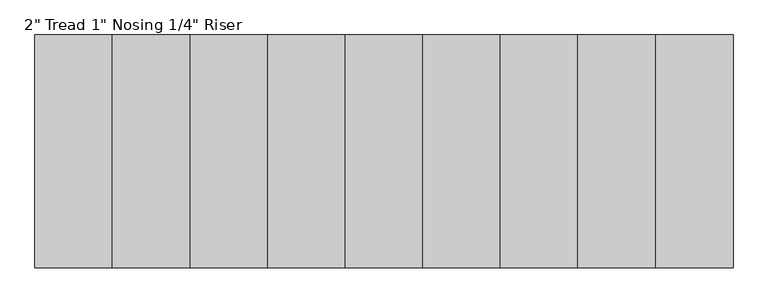
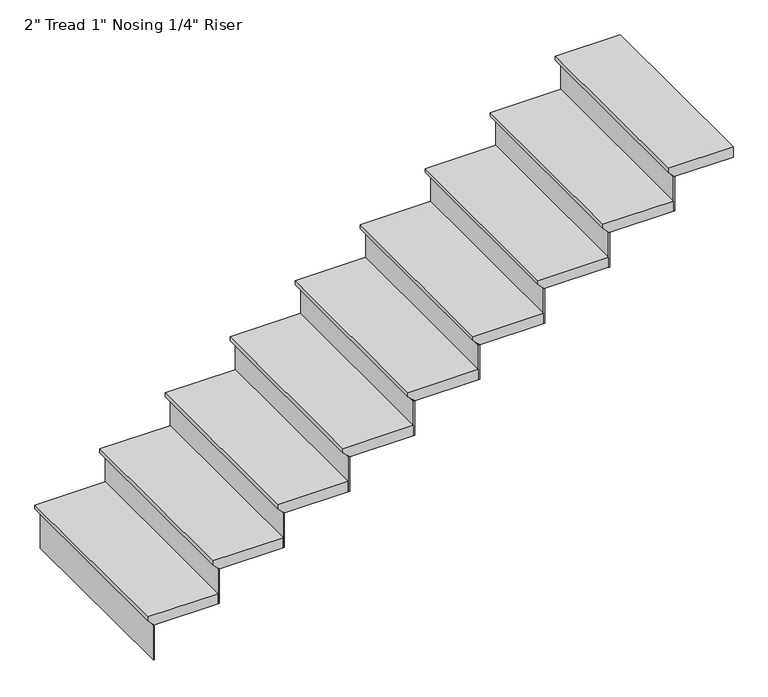
"""IFC4 building model written with IfcOpenShell, lengths in millimetres: stair flight geometry."""

from ifc_helpers import new_model, si_unit, frame, origin, place, context, project, spatial, polyline, outline, extrude, source, transform, mapped, element, save


def stair_flight_74c03164(model_context):
    return source(origin(), model_context, "Body", "SweptSolid", [
        extrude(outline(polyline([(1679.7734375, -8584.8920821), (1679.7734375, -8915.0920821), (1660.7234375, -8915.0920821), (1635.3234375, -8889.6920821), (1628.9734375, -8889.6920821), (1628.9734375, -8584.8920821), (1679.7734375, -8584.8920821)])), frame((0.0, 9649.0906648, 0.0), z_axis=(0.0, 1.0, 0.0), x_axis=(0.0, 0.0, 1.0)), (0.0, 0.0, 1.0), 914.4),
        extrude(outline(polyline([(-8883.3420821, 9649.0906648), (-8889.6920821, 9649.0906648), (-8889.6920821, 10563.4906648), (-8883.3420821, 10563.4906648), (-8883.3420821, 9649.0906648)])), frame((0.0, 0.0, 1457.9451172), z_axis=(0.0, 0.0, 1.0), x_axis=(1.0, 0.0, 0.0)), (0.0, 0.0, 1.0), 171.0283203),
        extrude(outline(polyline([(-8578.5420821, 9649.0906648), (-8584.8920821, 9649.0906648), (-8584.8920821, 10563.4906648), (-8578.5420821, 10563.4906648), (-8578.5420821, 9649.0906648)])), frame((0.0, 0.0, 1628.9734375), z_axis=(0.0, 0.0, 1.0), x_axis=(1.0, 0.0, 0.0)), (0.0, 0.0, 1.0), 171.0283203),
        extrude(outline(polyline([(1850.8017578, -8280.0920821), (1850.8017578, -8610.2920821), (1831.7517578, -8610.2920821), (1806.3517578, -8584.8920821), (1800.0017578, -8584.8920821), (1800.0017578, -8280.0920821), (1850.8017578, -8280.0920821)])), frame((0.0, 9649.0906648, 0.0), z_axis=(0.0, 1.0, 0.0), x_axis=(0.0, 0.0, 1.0)), (0.0, 0.0, 1.0), 914.4),
        extrude(outline(polyline([(-8273.7420821, 9649.0906648), (-8280.0920821, 9649.0906648), (-8280.0920821, 10563.4906648), (-8273.7420821, 10563.4906648), (-8273.7420821, 9649.0906648)])), frame((0.0, 0.0, 1800.0017578), z_axis=(0.0, 0.0, 1.0), x_axis=(1.0, 0.0, 0.0)), (0.0, 0.0, 1.0), 171.0283203),
        extrude(outline(polyline([(2021.8300781, -7975.2920821), (2021.8300781, -8305.4920821), (2002.7800781, -8305.4920821), (1977.3800781, -8280.0920821), (1971.0300781, -8280.0920821), (1971.0300781, -7975.2920821), (2021.8300781, -7975.2920821)])), frame((0.0, 9649.0906648, 0.0), z_axis=(0.0, 1.0, 0.0), x_axis=(0.0, 0.0, 1.0)), (0.0, 0.0, 1.0), 914.4),
        extrude(outline(polyline([(-7968.9420821, 9649.0906648), (-7975.2920821, 9649.0906648), (-7975.2920821, 10563.4906648), (-7968.9420821, 10563.4906648), (-7968.9420821, 9649.0906648)])), frame((0.0, 0.0, 1971.0300781), z_axis=(0.0, 0.0, 1.0), x_axis=(1.0, 0.0, 0.0)), (0.0, 0.0, 1.0), 171.0283203),
        extrude(outline(polyline([(2192.8583984, -7670.4920821), (2192.8583984, -8000.6920821), (2173.8083984, -8000.6920821), (2148.4083984, -7975.2920821), (2142.0583984, -7975.2920821), (2142.0583984, -7670.4920821), (2192.8583984, -7670.4920821)])), frame((0.0, 9649.0906648, 0.0), z_axis=(0.0, 1.0, 0.0), x_axis=(0.0, 0.0, 1.0)), (0.0, 0.0, 1.0), 914.4),
        extrude(outline(polyline([(-7664.1420821, 9649.0906648), (-7670.4920821, 9649.0906648), (-7670.4920821, 10563.4906648), (-7664.1420821, 10563.4906648), (-7664.1420821, 9649.0906648)])), frame((0.0, 0.0, 2142.0583984), z_axis=(0.0, 0.0, 1.0), x_axis=(1.0, 0.0, 0.0)), (0.0, 0.0, 1.0), 171.0283203),
        extrude(outline(polyline([(2363.8867188, -7365.6920821), (2363.8867188, -7695.8920821), (2344.8367188, -7695.8920821), (2319.4367188, -7670.4920821), (2313.0867188, -7670.4920821), (2313.0867188, -7365.6920821), (2363.8867188, -7365.6920821)])), frame((0.0, 9649.0906648, 0.0), z_axis=(0.0, 1.0, 0.0), x_axis=(0.0, 0.0, 1.0)), (0.0, 0.0, 1.0), 914.4),
        extrude(outline(polyline([(-7359.3420821, 9649.0906648), (-7365.6920821, 9649.0906648), (-7365.6920821, 10563.4906648), (-7359.3420821, 10563.4906648), (-7359.3420821, 9649.0906648)])), frame((0.0, 0.0, 2313.0867188), z_axis=(0.0, 0.0, 1.0), x_axis=(1.0, 0.0, 0.0)), (0.0, 0.0, 1.0), 171.0283203),
        extrude(outline(polyline([(2534.9150391, -7060.8920821), (2534.9150391, -7391.0920821), (2515.8650391, -7391.0920821), (2490.4650391, -7365.6920821), (2484.1150391, -7365.6920821), (2484.1150391, -7060.8920821), (2534.9150391, -7060.8920821)])), frame((0.0, 9649.0906648, 0.0), z_axis=(0.0, 1.0, 0.0), x_axis=(0.0, 0.0, 1.0)), (0.0, 0.0, 1.0), 914.4),
        extrude(outline(polyline([(-7054.5420821, 9649.0906648), (-7060.8920821, 9649.0906648), (-7060.8920821, 10563.4906648), (-7054.5420821, 10563.4906648), (-7054.5420821, 9649.0906648)])), frame((0.0, 0.0, 2484.1150391), z_axis=(0.0, 0.0, 1.0), x_axis=(1.0, 0.0, 0.0)), (0.0, 0.0, 1.0), 171.0283203),
        extrude(outline(polyline([(2705.9433594, -6756.0920821), (2705.9433594, -7086.2920821), (2686.8933594, -7086.2920821), (2661.4933594, -7060.8920821), (2655.1433594, -7060.8920821), (2655.1433594, -6756.0920821), (2705.9433594, -6756.0920821)])), frame((0.0, 9649.0906648, 0.0), z_axis=(0.0, 1.0, 0.0), x_axis=(0.0, 0.0, 1.0)), (0.0, 0.0, 1.0), 914.4),
        extrude(outline(polyline([(-6749.7420821, 9649.0906648), (-6756.0920821, 9649.0906648), (-6756.0920821, 10563.4906648), (-6749.7420821, 10563.4906648), (-6749.7420821, 9649.0906648)])), frame((0.0, 0.0, 2655.1433594), z_axis=(0.0, 0.0, 1.0), x_axis=(1.0, 0.0, 0.0)), (0.0, 0.0, 1.0), 171.0283203),
        extrude(outline(polyline([(2876.9716797, -6451.2920821), (2876.9716797, -6781.4920821), (2857.9216797, -6781.4920821), (2832.5216797, -6756.0920821), (2826.1716797, -6756.0920821), (2826.1716797, -6451.2920821), (2876.9716797, -6451.2920821)])), frame((0.0, 9649.0906648, 0.0), z_axis=(0.0, 1.0, 0.0), x_axis=(0.0, 0.0, 1.0)), (0.0, 0.0, 1.0), 914.4),
        extrude(outline(polyline([(-6444.9420821, 9649.0906648), (-6451.2920821, 9649.0906648), (-6451.2920821, 10563.4906648), (-6444.9420821, 10563.4906648), (-6444.9420821, 9649.0906648)])), frame((0.0, 0.0, 2826.1716797), z_axis=(0.0, 0.0, 1.0), x_axis=(1.0, 0.0, 0.0)), (0.0, 0.0, 1.0), 171.0283203),
        extrude(outline(polyline([(3048.0, -6171.8920821), (3048.0, -6476.6920821), (3028.95, -6476.6920821), (3003.55, -6451.2920821), (2997.2, -6451.2920821), (2997.2, -6171.8920821), (3048.0, -6171.8920821)])), frame((0.0, 9649.0906648, 0.0), z_axis=(0.0, 1.0, 0.0), x_axis=(0.0, 0.0, 1.0)), (0.0, 0.0, 1.0), 914.4),
    ])


if __name__ == "__main__":
    model = new_model("IFC4")
    model_context = context("Model", 3, world=origin())
    ifc_project = project(units=[si_unit("LENGTHUNIT", "METRE", prefix="MILLI")], contexts=[model_context])
    site = spatial("IfcSite", under=ifc_project)
    building = spatial("IfcBuilding", under=site)
    placement = place(None, origin())
    stair_flight_shape = stair_flight_74c03164(model_context)
    element("IfcStairFlight", 1, ObjectType="2\" Tread 1\" Nosing 1/4\" Riser", at=placement, inside=building, context=model_context, shape_type="MappedRepresentation", body=[
        mapped(stair_flight_shape, transform((0.0, 0.0, 0.0), x_axis=(1.0, 0.0, 0.0), y_axis=(0.0, 1.0, 0.0), z_axis=(0.0, 0.0, 1.0))),
    ])
    save(model, "model.ifc")
